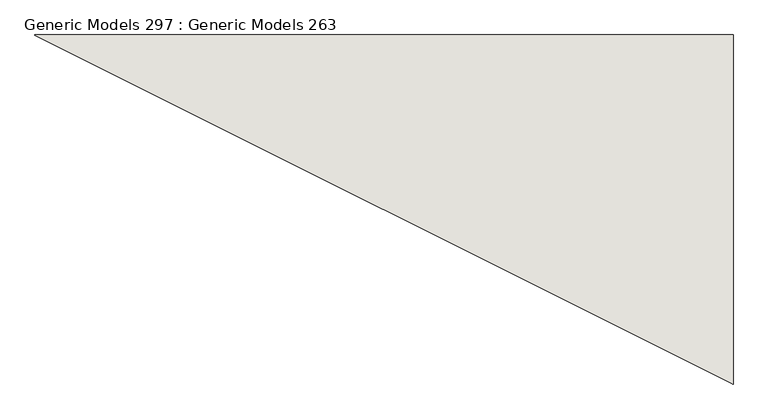
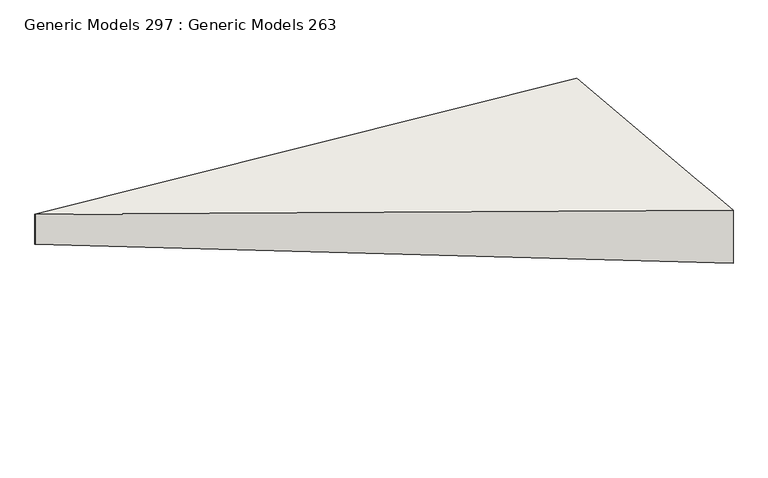
"""IFC4 building model written with IfcOpenShell, lengths in millimetres: wall geometry, Generic Models 297 : Generic Models 263."""

from ifc_helpers import new_model, si_unit, frame, origin, place, context, project, spatial, source, transform, mapped, element, save
from ifc_brep_helpers import plane_surface, spline_surface, advanced_brep


def generic_models_297_generic_models_263_bc1a45ca(model_context):
    return source(origin(), model_context, "Body", "AdvancedBrep", [
        advanced_brep(
        [(91554.5797726, -8256.6272578, 2.0699085), (91554.5797726, -8256.6272578, -314.8198762), (91554.5797726, -6732.6272578, -314.8198762), (91554.5797726, -6732.6272578, -137.0198762), (88506.5797726, -6733.7737439, 120.3150753), (88506.5797726, -6732.6272578, 120.3150753), (88506.5797726, -6732.6272578, -58.1173502), (88506.5797726, -6733.7737439, -58.1173502)],
        [
            (0, 1),
            (1, 2),
            (2, 3),
            (3, 0),
            (4, 5),
            (5, 6),
            (6, 7),
            (7, 4),
            (7, 1),
            (0, 4),
            (6, 2),
            (5, 3),
        ],
        [
            plane_surface(frame((91554.5797726, -7494.6272578, -191.14743), z_axis=(1.0, 0.0, 0.0), x_axis=(0.0, 0.0, -1.0))),
            plane_surface(frame((88506.5797726, -6733.2005009, 31.0988625), z_axis=(-1.0, 0.0, 0.0), x_axis=(0.0, 0.0, -1.0))),
            plane_surface(frame((88506.5797726, -6733.7737439, 31.0988625), z_axis=(-0.4469443881993885, -0.894561744016071, 0.0), x_axis=(0.0, 0.0, -1.0))),
            plane_surface(frame((88506.5797726, -6733.2005009, -58.1173502), z_axis=(-0.08392288197547094, 0.0, -0.9964722524390387), x_axis=(0.0, 1.0, 0.0))),
            plane_surface(frame((88506.5797726, -6732.6272578, 31.0988625), z_axis=(0.0, 1.0, 0.0), x_axis=(0.0, 0.0, 1.0))),
            spline_surface(1, 1, [[(88506.5797726, -6732.6272578, 120.3150753), (91554.5797726, -6732.6272578, -137.0198762)], [(88506.5797726, -6733.7737439, 120.3150753), (91554.5797726, -8256.6272578, 2.0699085)]], [2, 2], [2, 2], [0.0, 1.0], [0.0, 1.0]),
        ],
        [
            (0, [[1, 2, 3, 4]]),
            (1, [[5, 6, 7, 8]]),
            (2, [[-8, 9, -1, 10]]),
            (3, [[-7, 11, -2, -9]]),
            (4, [[-6, 12, -3, -11]]),
            (5, [[-5, -10, -4, -12]]),
        ],
    ),
    ])


if __name__ == "__main__":
    model = new_model("IFC4")
    model_context = context("Model", 3, world=origin())
    ifc_project = project(units=[si_unit("LENGTHUNIT", "METRE", prefix="MILLI")], contexts=[model_context])
    site = spatial("IfcSite", under=ifc_project)
    building = spatial("IfcBuilding", under=site)
    placement = place(None, origin())
    generic_models_297_generic_models_263_shape = generic_models_297_generic_models_263_bc1a45ca(model_context)
    element("IfcWall", 1, ObjectType="Generic Models 297 : Generic Models 263", at=placement, inside=building, context=model_context, shape_type="MappedRepresentation", body=[
        mapped(generic_models_297_generic_models_263_shape, transform((0.0, 0.0, 0.0), x_axis=(1.0, 0.0, 0.0), y_axis=(0.0, 1.0, 0.0), z_axis=(0.0, 0.0, 1.0))),
    ])
    save(model, "model.ifc")

# Revit data of these elements
# Element 1 (IfcWall, "Generic Models 297 : Generic Models 263")
#   Materials on its faces: "SLOPED - 7\" CONC."
# Materials
#   "SLOPED - 7\" CONC.": class "Concrete", colour RGB 191 191 191, transparency 0, Description = "Cast-in-place concrete", Cost = 0
